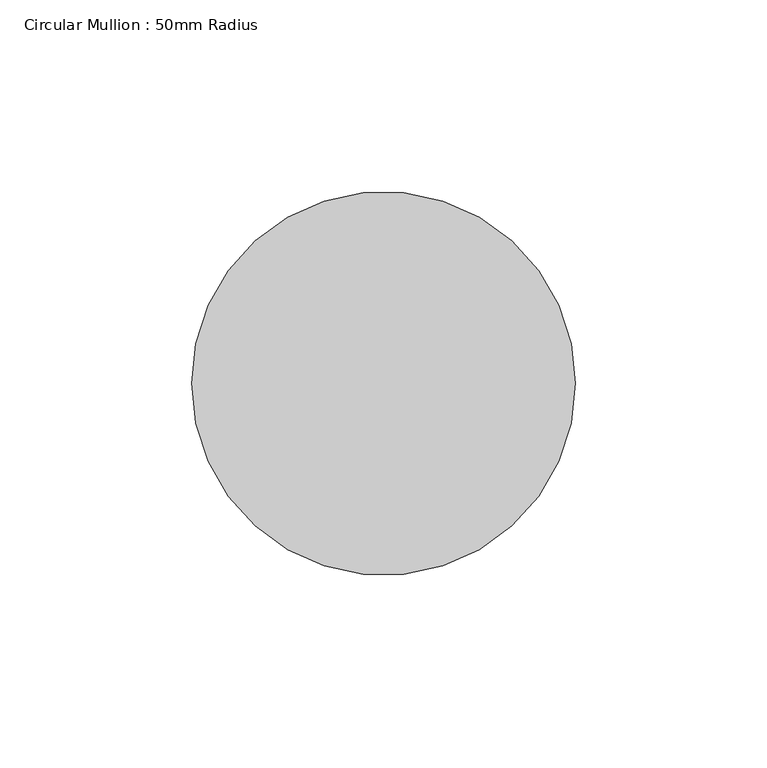
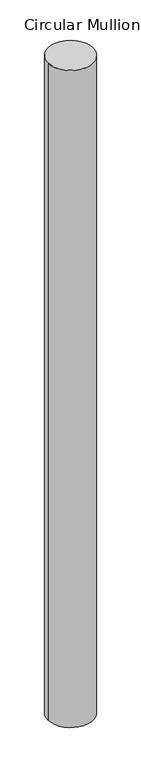
"""IFC4 building model written with IfcOpenShell, lengths in millimetres: member geometry, Circular Mullion : 50mm Radius."""

from ifc_helpers import new_model, si_unit, point, frame, origin, origin_2d, place, context, project, spatial, circle_curve, trimmed, segment, composite_curve, outline, extrude, source, transform, mapped, element, save


def circular_mullion_50mm_radius_7a7b4d10(model_context):
    return source(origin(), model_context, "Body", "SweptSolid", [
        extrude(outline(composite_curve([segment(trimmed(circle_curve(origin_2d(), 50.0), [point((50.0, 0.0))], [point((-50.0, 0.0))], False, "CARTESIAN"), True, "CONTINUOUS"), segment(trimmed(circle_curve(origin_2d(), 50.0), [point((-50.0, 0.0))], [point((50.0, 0.0))], False, "CARTESIAN"), True, "CONTINUOUS")], self_intersect=False)), frame((0.0, 0.0, -1530.0026482), z_axis=(0.0, 0.0, 1.0), x_axis=(1.0, 0.0, 0.0)), (0.0, 0.0, 1.0), 1530.0026482),
    ])


if __name__ == "__main__":
    model = new_model("IFC4")
    model_context = context("Model", 3, world=origin())
    ifc_project = project(units=[si_unit("LENGTHUNIT", "METRE", prefix="MILLI")], contexts=[model_context])
    site = spatial("IfcSite", under=ifc_project)
    building = spatial("IfcBuilding", under=site)
    placement = place(None, origin())
    circular_mullion_50mm_radius_shape = circular_mullion_50mm_radius_7a7b4d10(model_context)
    element("IfcMember", 1, ObjectType="Circular Mullion : 50mm Radius", at=placement, inside=building, context=model_context, shape_type="MappedRepresentation", body=[
        mapped(circular_mullion_50mm_radius_shape, transform((0.0, 0.0, 0.0), x_axis=(1.0, 0.0, 0.0), y_axis=(0.0, 1.0, 0.0), z_axis=(0.0, 0.0, 1.0))),
    ])
    save(model, "model.ifc")

# Revit data of these elements
# Type "Circular Mullion : 50mm Radius"
#   built-in parameter 1007350 = 0.164042 (stored number, unit not read)
# Element 1 (IfcMember, "Circular Mullion : 50mm Radius")
#   Materials on its faces: "Aluminium"
# Materials
#   "Aluminium": class "Metal", colour RGB 247 247 247, transparency 0, Description = "Aluminium 6061", Cost = 0
